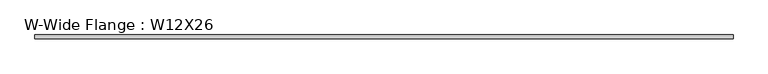
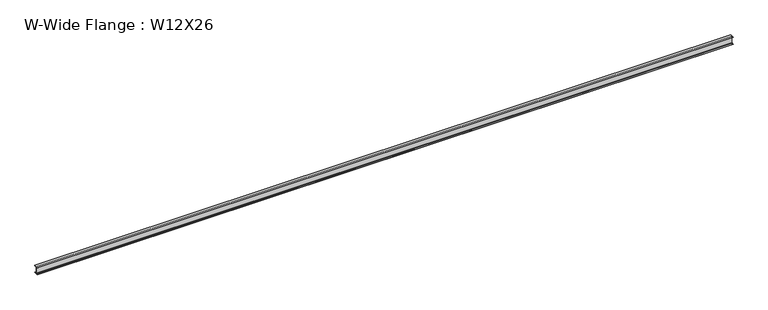
"""IFC4 building model written with IfcOpenShell, lengths in millimetres: beam geometry, W-Wide Flange : W12X26."""

from ifc_helpers import new_model, si_unit, point, frame, frame_2d, origin, place, context, project, spatial, polyline, circle_curve, trimmed, segment, composite_curve, outline, extrude, source, transform, mapped, element, save


def w_wide_flange_w12x26_70992f27(model_context):
    return source(origin(), model_context, "Body", "SweptSolid", [
        extrude(outline(composite_curve([segment(polyline([(82.4011719, -145.5539063), (82.4011719, -155.178125), (-82.4011719, -155.178125), (-82.4011719, -145.5539063), (-20.2902344, -145.5539063)]), True, "CONTINUOUS"), segment(trimmed(circle_curve(frame_2d((-20.2902344, -128.190625)), 17.3632812), [point((-20.2902344, -145.5539063))], [point((-2.9269531, -128.190625))], True, "CARTESIAN"), True, "CONTINUOUS"), segment(polyline([(-2.9269531, -128.190625), (-2.9269531, 128.190625)]), True, "CONTINUOUS"), segment(trimmed(circle_curve(frame_2d((-20.2902344, 128.190625)), 17.3632812), [point((-2.9269531, 128.190625))], [point((-20.2902344, 145.5539062))], True, "CARTESIAN"), True, "CONTINUOUS"), segment(polyline([(-20.2902344, 145.5539062), (-82.4011719, 145.5539062), (-82.4011719, 155.178125), (82.4011719, 155.178125), (82.4011719, 145.5539062), (20.2902344, 145.5539062)]), True, "CONTINUOUS"), segment(trimmed(circle_curve(frame_2d((20.2902344, 128.190625)), 17.3632812), [point((20.2902344, 145.5539062))], [point((2.9269531, 128.190625))], True, "CARTESIAN"), True, "CONTINUOUS"), segment(polyline([(2.9269531, 128.190625), (2.9269531, -128.190625)]), True, "CONTINUOUS"), segment(trimmed(circle_curve(frame_2d((20.2902344, -128.190625)), 17.3632812), [point((2.9269531, -128.190625))], [point((20.2902344, -145.5539063))], True, "CARTESIAN"), True, "CONTINUOUS"), segment(polyline([(20.2902344, -145.5539063), (82.4011719, -145.5539063)]), True, "CONTINUOUS")], self_intersect=False)), frame((-26596.6790574, 0.0, 0.0), z_axis=(1.0, 0.0, 0.0), x_axis=(0.0, 1.0, 0.0)), (0.0, 0.0, 1.0), 28844.2738475),
    ])


if __name__ == "__main__":
    model = new_model("IFC4")
    model_context = context("Model", 3, world=origin())
    ifc_project = project(units=[si_unit("LENGTHUNIT", "METRE", prefix="MILLI")], contexts=[model_context])
    site = spatial("IfcSite", under=ifc_project)
    building = spatial("IfcBuilding", under=site)
    placement = place(None, origin())
    w_wide_flange_w12x26_shape = w_wide_flange_w12x26_70992f27(model_context)
    element("IfcBeam", 1, ObjectType="W-Wide Flange : W12X26", at=placement, inside=building, context=model_context, shape_type="MappedRepresentation", body=[
        mapped(w_wide_flange_w12x26_shape, transform((0.0, 0.0, 0.0), x_axis=(1.0, 0.0, 0.0), y_axis=(0.0, 1.0, 0.0), z_axis=(0.0, 0.0, 1.0))),
    ])
    save(model, "model.ifc")

# Revit data of these elements
# Type "W-Wide Flange : W12X26"
#   Assembly Code = "B10"
#   W = 26
#   Length [instance default] = 5' - 0"
#   bf = 0' - 6 125/256"
#   d = 1' - 0 7/32"
#   k = 0' - 1 1/16"
#   k2 = 0' - 0 175/256"
#   tf = 0' - 0 97/256"
#   tw = 0' - 0 59/256"
#   A = 0.053125 SF
#   Structural Material [instance default] = none
